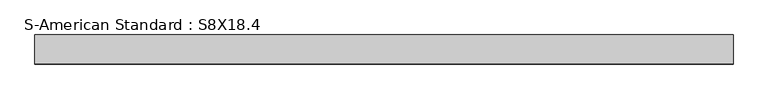
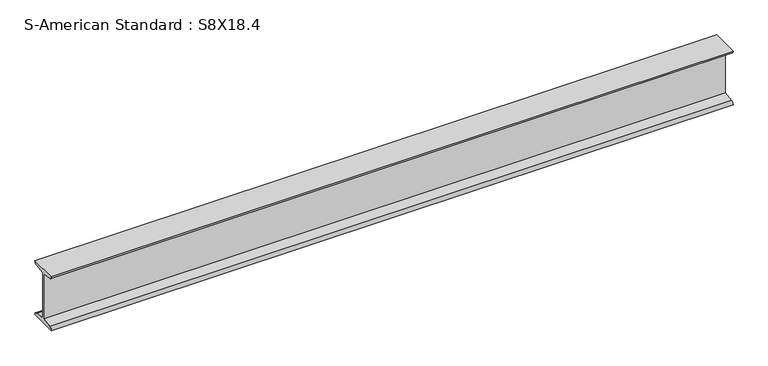
"""IFC4 building model written with IfcOpenShell, lengths in millimetres: beam geometry, S-American Standard : S8X18.4."""

from ifc_helpers import new_model, si_unit, point, frame, frame_2d, origin, place, context, project, spatial, polyline, circle_curve, trimmed, segment, composite_curve, outline, extrude, source, transform, mapped, element, save


def s_american_standard_s8x18_4_48e24ca1(model_context):
    return source(origin(), model_context, "Body", "SweptSolid", [
        extrude(outline(composite_curve([segment(polyline([(-50.8, 101.6), (50.8, 101.6)]), True, "CONTINUOUS"), segment(trimmed(circle_curve(frame_2d((40.005, 101.6)), 10.795), [point((50.8, 101.6))], [point((40.005, 90.805))], False, "CARTESIAN"), True, "CONTINUOUS"), segment(polyline([(40.005, 90.805), (3.4417, 85.0139422), (3.4417, -85.0139422), (40.005, -90.805)]), True, "CONTINUOUS"), segment(trimmed(circle_curve(frame_2d((40.005, -101.6)), 10.795), [point((40.005, -90.805))], [point((50.8, -101.6))], False, "CARTESIAN"), True, "CONTINUOUS"), segment(polyline([(50.8, -101.6), (-50.8, -101.6)]), True, "CONTINUOUS"), segment(trimmed(circle_curve(frame_2d((-40.005, -101.6)), 10.795), [point((-50.8, -101.6))], [point((-40.005, -90.805))], False, "CARTESIAN"), True, "CONTINUOUS"), segment(polyline([(-40.005, -90.805), (-3.4417, -85.0139422), (-3.4417, 85.0139422), (-40.005, 90.805)]), True, "CONTINUOUS"), segment(trimmed(circle_curve(frame_2d((-40.005, 101.6)), 10.795), [point((-40.005, 90.805))], [point((-50.8, 101.6))], False, "CARTESIAN"), True, "CONTINUOUS")], self_intersect=False)), frame((-1149.35, 0.0, 0.0), z_axis=(1.0, 0.0, 0.0), x_axis=(0.0, 1.0, 0.0)), (0.0, 0.0, 1.0), 2438.4),
    ])


if __name__ == "__main__":
    model = new_model("IFC4")
    model_context = context("Model", 3, world=origin())
    ifc_project = project(units=[si_unit("LENGTHUNIT", "METRE", prefix="MILLI")], contexts=[model_context])
    site = spatial("IfcSite", under=ifc_project)
    building = spatial("IfcBuilding", under=site)
    placement = place(None, origin())
    s_american_standard_s8x18_4_shape = s_american_standard_s8x18_4_48e24ca1(model_context)
    element("IfcBeam", 1, ObjectType="S-American Standard : S8X18.4", at=placement, inside=building, context=model_context, shape_type="MappedRepresentation", body=[
        mapped(s_american_standard_s8x18_4_shape, transform((0.0, 0.0, 0.0), x_axis=(1.0, 0.0, 0.0), y_axis=(0.0, 1.0, 0.0), z_axis=(0.0, 0.0, 1.0))),
    ])
    save(model, "model.ifc")

# Revit data of these elements
# Type "S-American Standard : S8X18.4"
#   Assembly Code = "B10"
#   W = 18.4
#   Length [instance default] = 5' - 0"
#   bf = 0' - 4"
#   d = 0' - 8"
#   k = 0' - 1"
#   tf = 0' - 0.425"
#   tw = 0' - 0.271"
#   A = 0.0375 SF
#   Structural Material [instance default] = Steel ASTM A572
# Element 1 (IfcBeam, "S-American Standard : S8X18.4")
#   Materials on its faces: "Steel ASTM A572"
# Materials
#   "Steel ASTM A572": class "Metal", colour RGB 247 247 247, transparency 0, Description = "Structural steel, high strength low alloy, ASTM - A572 - 50", Cost = 0
